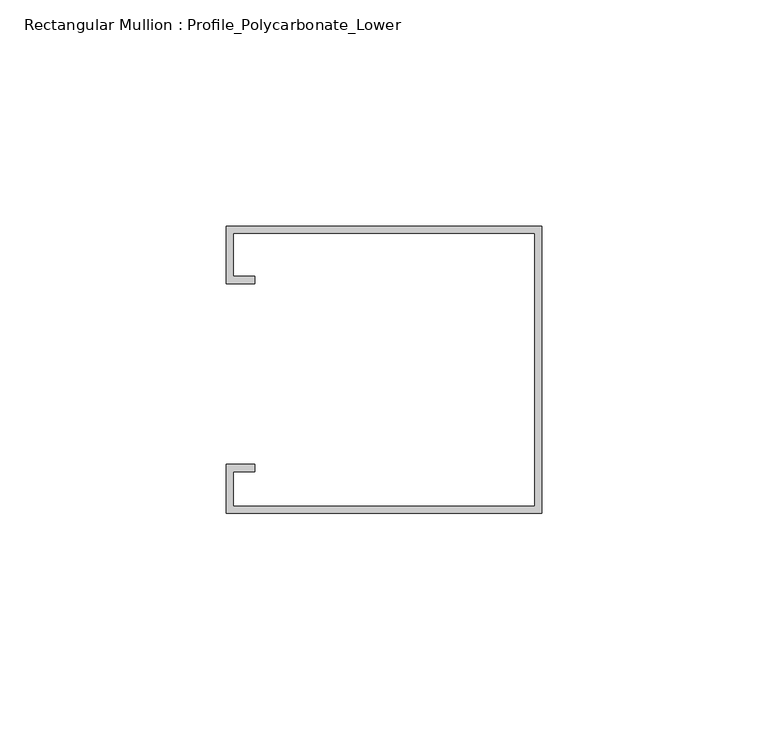
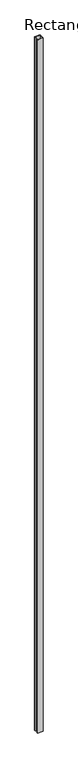
"""IFC4 building model written with IfcOpenShell, lengths in millimetres: member geometry, Rectangular Mullion : Profile_Polycarbonate_Lower."""

import ifcopenshell
import ifcopenshell.guid

model = None  # the IFC model being written
_history = None  # IfcOwnerHistory: only IFC2X3 demands one
_inside = {}  # id of a spatial element -> (the spatial element, [elements in it])
_under = {}  # id of a project, library or spatial element -> (it, [spatial elements below it])
_declared = {}  # id of a project -> (the project, [libraries it declares])
_typed = {}  # id of a type object -> (the type object, [elements of that type])
_made_of = {}  # id of a material, layer set ... -> (it, [elements and type objects made of it])


def new_model(schema):
    """Start an empty IFC model of exactly this schema.

    Asked for "IFC4X3", IfcOpenShell would pick the latest addendum, in which some entities
    have other attributes; the version numbers below select the first issue.
    IFC2X3 requires an IfcOwnerHistory on every rooted entity: one is made here for all.
    """
    global model, _history
    if schema == "IFC4X3":
        model = ifcopenshell.file(schema_version=(4, 3, 0, 0))
    else:
        model = ifcopenshell.file(schema=schema)
    _inside.clear()
    _under.clear()
    _declared.clear()
    _typed.clear()
    _made_of.clear()
    _history = None
    if model.schema == "IFC2X3":
        org = make("IfcOrganization", Name="unknown")
        user = make(
            "IfcPersonAndOrganization",
            ThePerson=make("IfcPerson", FamilyName="unknown"),
            TheOrganization=org,
        )
        app = make(
            "IfcApplication",
            ApplicationDeveloper=org,
            Version="unknown",
            ApplicationFullName="unknown",
            ApplicationIdentifier="unknown",
        )
        _history = make(
            "IfcOwnerHistory",
            OwningUser=user,
            OwningApplication=app,
            ChangeAction="ADDED",
            CreationDate=0,
        )
    return model


def make(cls, **values):
    """One entity of the class cls with the attributes given. An attribute that is None is left unset."""
    return model.create_entity(
        cls, **{name: value for name, value in values.items() if value is not None}
    )


def rooted(cls, **values):
    """An entity with a GlobalId (a new one), such as an element, a storey or a relation."""
    return make(cls, GlobalId=ifcopenshell.guid.new(), OwnerHistory=_history, **values)


def si_unit(unit_type, name, prefix=None):
    """IfcSIUnit, for example si_unit("LENGTHUNIT", "METRE", prefix="MILLI")."""
    return make("IfcSIUnit", UnitType=unit_type, Prefix=prefix, Name=name)


def assignment(units):
    """IfcUnitAssignment: the units of a project."""
    return None if units is None else make("IfcUnitAssignment", Units=units)


def point(xyz):
    """IfcCartesianPoint."""
    return None if xyz is None else make("IfcCartesianPoint", Coordinates=xyz)


def direction(xyz):
    """IfcDirection."""
    return None if xyz is None else make("IfcDirection", DirectionRatios=xyz)


def frame(location, z_axis=None, x_axis=None):
    """IfcAxis2Placement3D, a coordinate frame: its origin and axes. An axis left out is left unset."""
    return make(
        "IfcAxis2Placement3D",
        Location=point(location),
        Axis=direction(z_axis),
        RefDirection=direction(x_axis),
    )


def origin():
    """The frame at (0, 0, 0) with its axes left unset."""
    return frame((0.0, 0.0, 0.0))


def place(relative_to, where):
    """IfcLocalPlacement: puts the frame where relative to a parent placement (None: the world)."""
    return make(
        "IfcLocalPlacement", PlacementRelTo=relative_to, RelativePlacement=where
    )


def context(
    kind, dimensions, precision=None, world=None, true_north=None, identifier=None
):
    """IfcGeometricRepresentationContext, for example the 3D "Model" context."""
    return make(
        "IfcGeometricRepresentationContext",
        ContextIdentifier=identifier,
        ContextType=kind,
        CoordinateSpaceDimension=dimensions,
        Precision=precision,
        WorldCoordinateSystem=world,
        TrueNorth=true_north,
    )


def project(units=None, contexts=None):
    """IfcProject with its units and contexts."""
    return rooted(
        "IfcProject",
        Name="project",
        RepresentationContexts=contexts,
        UnitsInContext=assignment(units),
    )


def spatial(cls, under=None, at=None, **own):
    """A site, building, storey or space (cls), placed at a placement, below another one or the project."""
    s = rooted(cls, ObjectPlacement=at, **own)
    if under is not None:
        _under.setdefault(under.id(), (under, []))[1].append(s)
    return s


def polyline(points):
    """IfcPolyline through the points."""
    return make("IfcPolyline", Points=[point(p) for p in points])


def outline(outer, holes=None, kind="AREA"):
    """IfcArbitraryClosedProfileDef: a profile drawn as a closed curve; with holes, ...WithVoids."""
    if holes is None:
        return make("IfcArbitraryClosedProfileDef", ProfileType=kind, OuterCurve=outer)
    return make(
        "IfcArbitraryProfileDefWithVoids",
        ProfileType=kind,
        OuterCurve=outer,
        InnerCurves=holes,
    )


def extrude(swept, where, along, depth):
    """IfcExtrudedAreaSolid: the profile swept, set in the frame where, extruded along a direction by depth."""
    return make(
        "IfcExtrudedAreaSolid",
        SweptArea=swept,
        Position=where,
        ExtrudedDirection=direction(along),
        Depth=depth,
    )


def shape(context_of_items, identifier, shape_type, items):
    """IfcShapeRepresentation: the items that make up one representation, for example the "Body"."""
    return make(
        "IfcShapeRepresentation",
        ContextOfItems=context_of_items,
        RepresentationIdentifier=identifier,
        RepresentationType=shape_type,
        Items=items,
    )


def source(mapping_origin, context_of_items, identifier, shape_type, items):
    """IfcRepresentationMap: a shape defined once, which mapped items show again and again."""
    return make(
        "IfcRepresentationMap",
        MappingOrigin=mapping_origin,
        MappedRepresentation=shape(context_of_items, identifier, shape_type, items),
    )


def transform(
    local_origin,
    x_axis=None,
    y_axis=None,
    z_axis=None,
    scale=None,
    scale2=None,
    scale3=None,
    uniform=True,
):
    """IfcCartesianTransformationOperator3D, or its non-uniform kind. x_axis, y_axis, z_axis: its Axis1, 2, 3."""
    if uniform:
        return make(
            "IfcCartesianTransformationOperator3D",
            Axis1=direction(x_axis),
            Axis2=direction(y_axis),
            LocalOrigin=point(local_origin),
            Scale=scale,
            Axis3=direction(z_axis),
        )
    return make(
        "IfcCartesianTransformationOperator3DnonUniform",
        Axis1=direction(x_axis),
        Axis2=direction(y_axis),
        LocalOrigin=point(local_origin),
        Scale=scale,
        Axis3=direction(z_axis),
        Scale2=scale2,
        Scale3=scale3,
    )


def mapped(mapping_source, mapping_target):
    """IfcMappedItem: shows the shape of a source again, moved by a transform."""
    return make(
        "IfcMappedItem", MappingSource=mapping_source, MappingTarget=mapping_target
    )


def made_of(thing, what):
    """Note that an element or type object is made of a material, layer set ...; save() writes the relation."""
    if what is not None:
        _made_of.setdefault(what.id(), (what, []))[1].append(thing)
    return thing


def element(
    cls,
    number,
    at=None,
    inside=None,
    cuts=None,
    type_object=None,
    material=None,
    context=None,
    identifier="Body",
    shape_type=None,
    held_by="IfcProductDefinitionShape",
    body=None,
    shapes=None,
    **own,
):
    """One element of the class cls, such as IfcWall. Its Tag is "e" and its number.

    at: its placement. inside: the storey or other place that contains it. cuts: it is an
    opening in that element (IfcRelVoidsElement). A single representation is given by context,
    identifier, shape_type and body (its items); several are given by shapes. held_by: the class
    of the entity that holds the representations. save() writes the other relations.
    """
    e = rooted(cls, Tag="e%d" % number, ObjectPlacement=at, **own)
    if body is not None:
        shapes = [shape(context, identifier, shape_type, body)]
    if shapes is not None:
        e.Representation = make(held_by, Representations=shapes)
    if inside is not None:
        _inside.setdefault(inside.id(), (inside, []))[1].append(e)
    if cuts is not None:
        rooted(
            "IfcRelVoidsElement", RelatingBuildingElement=cuts, RelatedOpeningElement=e
        )
    if type_object is not None:
        _typed.setdefault(type_object.id(), (type_object, []))[1].append(e)
    return made_of(e, material)


def aggregate(whole, parts):
    """IfcRelAggregates: a whole, such as a stair, and the parts it consists of."""
    return rooted("IfcRelAggregates", RelatingObject=whole, RelatedObjects=parts)


def save(model, path):
    """Write the relations noted so far, then the file.

    IfcRelAggregates (storeys below a building ...), IfcRelContainedInSpatialStructure (elements
    in a storey), IfcRelDefinesByType, IfcRelAssociatesMaterial and IfcRelDeclares: one each for
    every whole, place, type object, material and project.
    """
    for whole, parts in _under.values():
        aggregate(whole, parts)
    for where, things in _inside.values():
        rooted(
            "IfcRelContainedInSpatialStructure",
            RelatedElements=things,
            RelatingStructure=where,
        )
    for kind, things in _typed.values():
        rooted("IfcRelDefinesByType", RelatedObjects=things, RelatingType=kind)
    for what, things in _made_of.values():
        rooted("IfcRelAssociatesMaterial", RelatedObjects=things, RelatingMaterial=what)
    for by, libraries in _declared.values():
        rooted("IfcRelDeclares", RelatingContext=by, RelatedDefinitions=libraries)
    model.write(path)


def rectangular_mullion_profile_polycarbonate_lower_b602086c(model_context):
    return source(origin(), model_context, "Body", "SweptSolid", [
        extrude(outline(polyline([(0.0, 32.7), (0.0, -30.8), (-69.85, -30.8), (-69.85, -20.0), (-63.5, -20.0), (-63.5, -21.5875), (-68.2625, -21.5875), (-68.2625, -29.2125), (-1.5875, -29.2125), (-1.5875, 31.1125), (-68.2625, 31.1125), (-68.2625, 21.5875), (-63.5, 21.5875), (-63.5, 20.0), (-69.85, 20.0), (-69.85, 32.7), (0.0, 32.7)])), frame((0.0, 0.0, -9170.9875), z_axis=(0.0, 0.0, 1.0), x_axis=(1.0, 0.0, 0.0)), (0.0, 0.0, 1.0), 9170.9875),
    ])


if __name__ == "__main__":
    model = new_model("IFC4")
    model_context = context("Model", 3, world=origin())
    ifc_project = project(units=[si_unit("LENGTHUNIT", "METRE", prefix="MILLI")], contexts=[model_context])
    site = spatial("IfcSite", under=ifc_project)
    building = spatial("IfcBuilding", under=site)
    placement = place(None, origin())
    rectangular_mullion_profile_polycarbonate_lower_shape = rectangular_mullion_profile_polycarbonate_lower_b602086c(model_context)
    element("IfcMember", 1, ObjectType="Rectangular Mullion : Profile_Polycarbonate_Lower", at=placement, inside=building, context=model_context, shape_type="MappedRepresentation", body=[
        mapped(rectangular_mullion_profile_polycarbonate_lower_shape, transform((0.0, 0.0, 0.0), x_axis=(1.0, 0.0, 0.0), y_axis=(0.0, 1.0, 0.0), z_axis=(0.0, 0.0, 1.0))),
    ])
    save(model, "model.ifc")

# Revit data of these elements
# Type "Rectangular Mullion : Profile_Polycarbonate_Lower"
#   built-in parameter 1007322 = 0.208333 (stored number, unit not read)
#   built-in parameter 1007321 = 0 (stored number, unit not read)
#   built-in parameter 1007320 = 0.00520833 (stored number, unit not read)
# Element 1 (IfcMember, "Rectangular Mullion : Profile_Polycarbonate_Lower")
#   Materials on its faces: "ALUMINUM PROFILE AT POLYCARBONATE PANEL"
# Materials
#   "ALUMINUM PROFILE AT POLYCARBONATE PANEL": class "Metal", colour RGB 244 244 244, transparency 0, Description = "Aluminum 6061", Cost = 0
